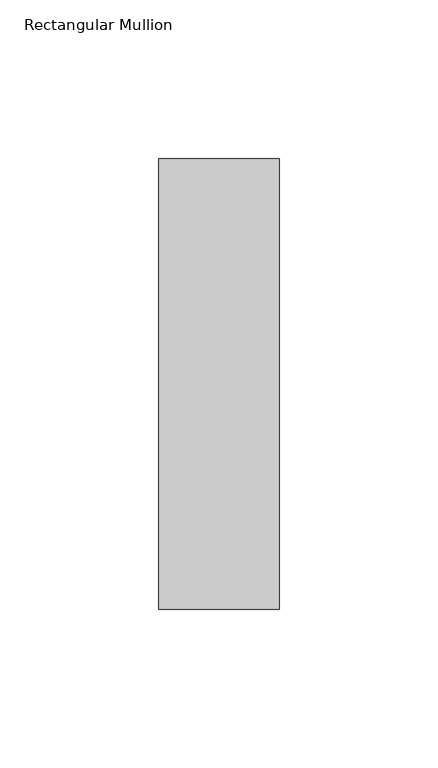
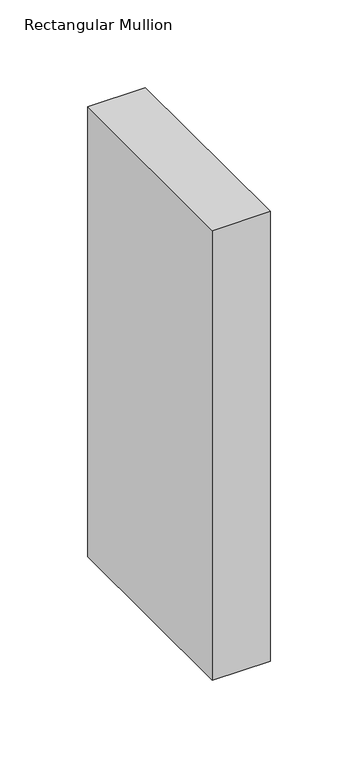
"""IFC4 building model written with IfcOpenShell, lengths in millimetres: member geometry, Rectangular Mullion : NLRS_21_CWM_hsb-regel 38x142_gen_rsf."""

from ifc_helpers import new_model, si_unit, frame, origin, place, context, project, spatial, polyline, outline, extrude, source, transform, mapped, element, save


def rectangular_mullion_6d68dd6a(model_context):
    return source(origin(), model_context, "Body", "SweptSolid", [
        extrude(outline(polyline([(0.0, -71.0), (-38.0, -71.0), (-38.0, 71.0), (0.0, 71.0), (0.0, -71.0)])), frame((0.0, 0.0, -312.8441061), z_axis=(0.0, 0.0, 1.0), x_axis=(1.0, 0.0, 0.0)), (0.0, 0.0, 1.0), 312.8441061),
    ])


if __name__ == "__main__":
    model = new_model("IFC4")
    model_context = context("Model", 3, world=origin())
    ifc_project = project(units=[si_unit("LENGTHUNIT", "METRE", prefix="MILLI")], contexts=[model_context])
    site = spatial("IfcSite", under=ifc_project)
    building = spatial("IfcBuilding", under=site)
    placement = place(None, origin())
    rectangular_mullion_shape = rectangular_mullion_6d68dd6a(model_context)
    element("IfcMember", 1, ObjectType="Rectangular Mullion : NLRS_21_CWM_hsb-regel 38x142_gen_rsf", at=placement, inside=building, context=model_context, shape_type="MappedRepresentation", body=[
        mapped(rectangular_mullion_shape, transform((0.0, 0.0, 0.0), x_axis=(1.0, 0.0, 0.0), y_axis=(0.0, 1.0, 0.0), z_axis=(0.0, 0.0, 1.0))),
    ])
    save(model, "model.ifc")

# Revit data of these elements
# Type "Rectangular Mullion : NLRS_21_CWM_hsb-regel 38x142_gen_rsf"
#   Export Type to IFC As = "IfcWall"
#   Type IfcGUID = "07M7mRoiH1CR8m_RSKIwpF"
#   Assembly Code = "21.10"
#   built-in parameter 1007322 = 0.465879 (stored number, unit not read)
#   built-in parameter 1007321 = 0.062336 (stored number, unit not read)
#   built-in parameter 1007320 = 0.062336 (stored number, unit not read)
# Element 1 (IfcMember, "Rectangular Mullion : NLRS_21_CWM_hsb-regel 38x142_gen_rsf")
#   Materials on its faces: "NLRS_i2_hout naaldhout vuren_gen_rsf"
# Materials
#   "NLRS_i2_hout naaldhout vuren_gen_rsf": class "I - Hout", colour RGB 234 199 147, transparency 0, Keynote = "i2", Manufacturer = "Revit Standards Foundation", URL = "www.revitstandards.org", Description = "hout vuren", Cost = 0
